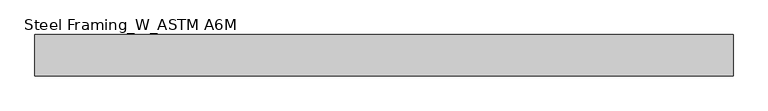
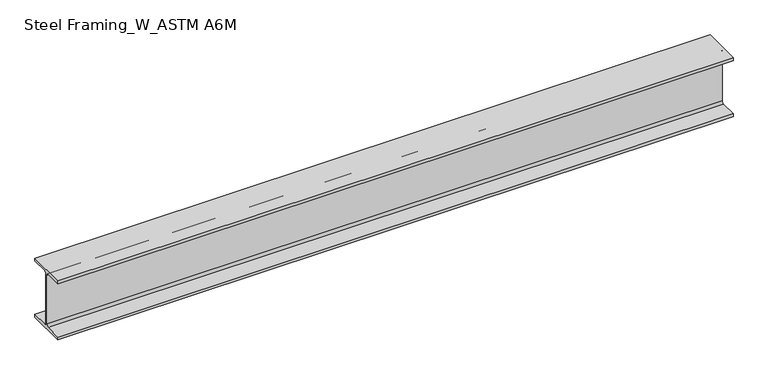
"""IFC4 building model written with IfcOpenShell, lengths in millimetres: beam geometry, Steel Framing_W_ASTM A6M : H_SB_AR_S02_W200x31.3_B6."""

from ifc_helpers import new_model, si_unit, point, frame, frame_2d, origin, place, context, project, spatial, polyline, circle_curve, trimmed, segment, composite_curve, outline, extrude, source, transform, mapped, element, save


def steel_framing_w_astm_a6m_9f313648(model_context):
    return source(origin(), model_context, "Body", "SweptSolid", [
        extrude(outline(composite_curve([segment(polyline([(67.0, -94.8), (67.0, -105.0), (-67.0, -105.0), (-67.0, -94.8), (-10.775, -94.8)]), True, "CONTINUOUS"), segment(trimmed(circle_curve(frame_2d((-10.775, -87.2)), 7.6), [point((-10.775, -94.8))], [point((-3.175, -87.2))], True, "CARTESIAN"), True, "CONTINUOUS"), segment(polyline([(-3.175, -87.2), (-3.175, 87.2)]), True, "CONTINUOUS"), segment(trimmed(circle_curve(frame_2d((-10.775, 87.2)), 7.6), [point((-3.175, 87.2))], [point((-10.775, 94.8))], True, "CARTESIAN"), True, "CONTINUOUS"), segment(polyline([(-10.775, 94.8), (-67.0, 94.8), (-67.0, 105.0), (67.0, 105.0), (67.0, 94.8), (10.775, 94.8)]), True, "CONTINUOUS"), segment(trimmed(circle_curve(frame_2d((10.775, 87.2)), 7.6), [point((10.775, 94.8))], [point((3.175, 87.2))], True, "CARTESIAN"), True, "CONTINUOUS"), segment(polyline([(3.175, 87.2), (3.175, -87.2)]), True, "CONTINUOUS"), segment(trimmed(circle_curve(frame_2d((10.775, -87.2)), 7.6), [point((3.175, -87.2))], [point((10.775, -94.8))], True, "CARTESIAN"), True, "CONTINUOUS"), segment(polyline([(10.775, -94.8), (67.0, -94.8)]), True, "CONTINUOUS")], self_intersect=False)), frame((-1135.8, 0.0, 0.0), z_axis=(1.0, 0.0, 0.0), x_axis=(0.0, 1.0, 0.0)), (0.0, 0.0, 1.0), 2271.6),
    ])


if __name__ == "__main__":
    model = new_model("IFC4")
    model_context = context("Model", 3, world=origin())
    ifc_project = project(units=[si_unit("LENGTHUNIT", "METRE", prefix="MILLI")], contexts=[model_context])
    site = spatial("IfcSite", under=ifc_project)
    building = spatial("IfcBuilding", under=site)
    placement = place(None, origin())
    steel_framing_w_astm_a6m_shape = steel_framing_w_astm_a6m_9f313648(model_context)
    element("IfcBeam", 1, ObjectType="Steel Framing_W_ASTM A6M : H_SB_AR_S02_W200x31.3_B6", at=placement, inside=building, context=model_context, shape_type="MappedRepresentation", body=[
        mapped(steel_framing_w_astm_a6m_shape, transform((0.0, 0.0, 0.0), x_axis=(1.0, 0.0, 0.0), y_axis=(0.0, 1.0, 0.0), z_axis=(0.0, 0.0, 1.0))),
    ])
    save(model, "model.ifc")

# Revit data of these elements
# Type "Steel Framing_W_ASTM A6M : H_SB_AR_S02_W200x31.3_B6"
#   Type Mark = "B6"
#   Section Name Key = "W8x21"
#   Width = 13.4 cm
#   Web Thickness = 0.635 cm
#   Web Fillet = 0.76 cm
#   Warping Constant = 40800.0 cm⁶
#   Torsional Moment of Inertia = 11.70 cm⁴
#   Section Area = 39.7 cm²
#   Plastic Modulus weak axis = 93.2 cm³
#   Plastic Modulus strong axis = 334.0 cm³
#   Perimeter = 0.93 m²/m
#   Nominal Weight = 31.30 kgf/m
#   Moment of Inertia weak axis = 407.00 cm⁴
#   Moment of Inertia strong axis = 3130.00 cm⁴
#   Height = 21.0 cm
#   Flange Thickness = 1.02 cm
#   Elastic Modulus weak axis = 60.8 cm³
#   Elastic Modulus strong axis = 298.0 cm³
#   Centroid Vertical = 10.5 cm
#   Centroid Horizontal = 6.7 cm
#   Length [instance default] = 1500 mm
#   Structural Material [instance default] = Steel, 45-345
#   Bolt Spacing = 0
#   Assembly Code = ""
# Element 1 (IfcBeam, "Steel Framing_W_ASTM A6M : H_SB_AR_S02_W200x31.3_B6")
#   Materials on its faces: "Steel, 45-345"
# Materials
#   "Steel, 45-345": class "Metal", colour RGB 189 187 185, transparency 0, Description = "Steel 345 MPa", Cost = 0
